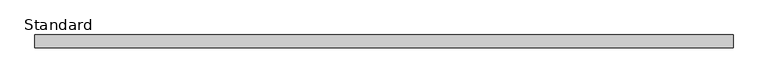
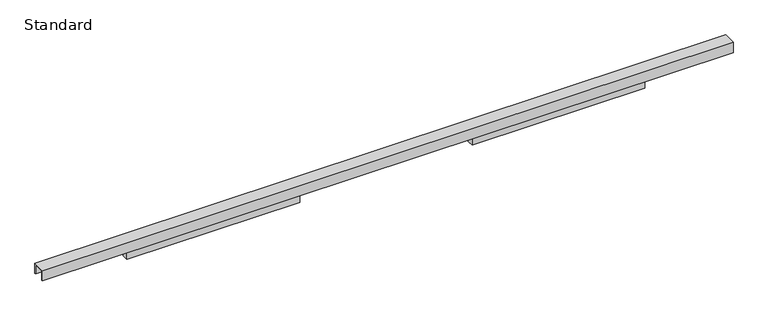
"""IFC4 building model written with IfcOpenShell, lengths in millimetres: plate geometry, Türelement 2-flg - Schiebeflügel : Standard."""

from ifc_helpers import new_model, si_unit, frame, origin, origin_with_axes, place, context, project, spatial, polyline, outline, extrude, source, transform, mapped, element, save


def standard_af362adf(model_context):
    return source(origin(), model_context, "Body", "SweptSolid", [
        extrude(outline(polyline([(1200.0, -100.0), (1200.0, -130.0), (400.0, -130.0), (400.0, -100.0), (1200.0, -100.0)])), origin_with_axes(), (0.0, 0.0, 1.0), 43.984045),
        extrude(outline(polyline([(-400.0, -100.0), (-400.0, -130.0), (-1200.0, -130.0), (-1200.0, -100.0), (-400.0, -100.0)])), origin_with_axes(), (0.0, 0.0, 1.0), 43.984045),
        extrude(outline(polyline([(-140.0, 88.984045), (-140.0, 43.984045), (-145.0, 43.984045), (-145.0, 93.984045), (-85.0, 93.984045), (-85.0, 43.984045), (-90.0, 43.984045), (-90.0, 88.984045), (-140.0, 88.984045)])), frame((-1600.0, 0.0, 0.0), z_axis=(1.0, 0.0, 0.0), x_axis=(0.0, 1.0, 0.0)), (0.0, 0.0, 1.0), 3200.0),
    ])


if __name__ == "__main__":
    model = new_model("IFC4")
    model_context = context("Model", 3, world=origin())
    ifc_project = project(units=[si_unit("LENGTHUNIT", "METRE", prefix="MILLI")], contexts=[model_context])
    site = spatial("IfcSite", under=ifc_project)
    building = spatial("IfcBuilding", under=site)
    placement = place(None, origin())
    standard_shape = standard_af362adf(model_context)
    element("IfcPlate", 1, ObjectType="Türelement 2-flg - Schiebeflügel : Standard", at=placement, inside=building, context=model_context, shape_type="MappedRepresentation", body=[
        mapped(standard_shape, transform((0.0, 0.0, 0.0), x_axis=(1.0, 0.0, 0.0), y_axis=(0.0, 1.0, 0.0), z_axis=(0.0, 0.0, 1.0))),
    ])
    save(model, "model.ifc")

# Revit data of these elements
# Type "Türelement 2-flg - Schiebeflügel : Standard"
#   Construction Type Id = "GSP4R"
#   Analytic Construction = "1/8 Zoll Pilkington-Verglasung einfach"
#   Visual Light Transmittance = 0.9
#   Thermal Resistance (R) = 0.270117 (m²·K)/W
#   Solar Heat Gain Coefficient = 0.86
#   Öffnungswert [instance default] = 0.400 m
#   Heat Transfer Coefficient (U) = 6.7069 W/(m²·K)
#   Länge Schiene [instance default] = 3.200 m
#   Halbe Breite [instance default] = 0.800 m
#   Versatz zur Achse [instance default] = 0.100 m
#   Gesamtbreite Tür [instance default] = 1.600 m
#   Schiene anzeigen [instance default] = yes
#   Prozent [instance default] = 50
#   Geöffnet in % [instance default] = 50
#   Schiene [instance default] = none
#   Tür [instance default] = none
# Element 1 (IfcPlate, "Türelement 2-flg - Schiebeflügel : Standard")
#   Materials on its faces: "Glas"
# Materials
#   "Glas": class "Glas", colour RGB 0 0 255, transparency 0.75, Comments = "Render-Darstellung nicht aktualisiert ", Cost = 0
